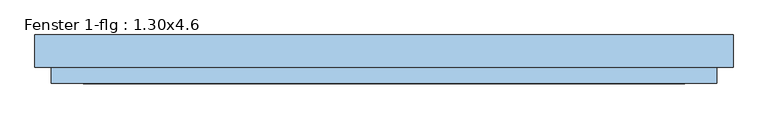
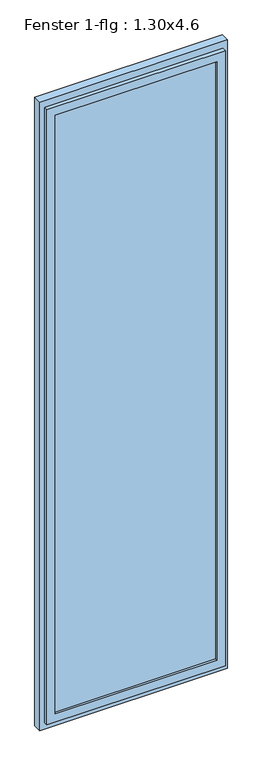
"""IFC4 building model written with IfcOpenShell, lengths in millimetres: window geometry, Fenster 1-flg : 1.30x4.6."""

from ifc_helpers import new_model, si_unit, frame, origin, place, context, project, spatial, polyline, outline, extrude, faceted_brep, source, transform, mapped, element, save


def fenster_1_flg_1_30x4_6_5ba6886f(model_context):
    return source(origin(), model_context, "Body", "SolidModel", [
        extrude(outline(polyline([(5600.0, 650.0), (5600.0, -650.0), (1000.0, -650.0), (1000.0, 650.0), (5600.0, 650.0)]), holes=[polyline([(5520.0, 590.0), (1080.0, 590.0), (1080.0, -590.0), (5520.0, -590.0), (5520.0, 590.0)])]), frame((0.0, -15.0, 0.0), z_axis=(0.0, 1.0, 0.0), x_axis=(0.0, 0.0, 1.0)), (0.0, 0.0, 1.0), 60.0),
        faceted_brep([(620.0, -15.0, 5550.0), (620.0, -45.0, 5550.0), (620.0, -45.0, 1050.0), (620.0, -15.0, 1050.0), (-620.0, -45.0, 5550.0), (-620.0, -45.0, 1050.0), (560.0, -45.0, 1110.0), (-560.0, -45.0, 1110.0), (-560.0, -45.0, 5490.0), (560.0, -45.0, 5490.0), (-620.0, -15.0, 1050.0), (-620.0, -15.0, 5550.0), (590.0, -15.0, 5520.0), (-590.0, -15.0, 5520.0), (-590.0, -15.0, 1080.0), (590.0, -15.0, 1080.0), (590.0, 15.0, 5520.0), (590.0, 15.0, 1080.0), (-590.0, 15.0, 1080.0), (-590.0, 15.0, 5520.0), (560.0, 15.0, 5490.0), (-560.0, 15.0, 5490.0), (-560.0, 15.0, 1110.0), (560.0, 15.0, 1110.0)], [[[0, 1, 2, 3]], [[1, 4, 5, 2], [6, 7, 8, 9]], [[3, 2, 5, 10]], [[3, 10, 11, 0], [12, 13, 14, 15]], [[16, 12, 15, 17]], [[17, 15, 14, 18]], [[17, 18, 19, 16], [20, 21, 22, 23]], [[9, 20, 23, 6]], [[6, 23, 22, 7]], [[10, 5, 4, 11]], [[18, 14, 13, 19]], [[7, 22, 21, 8]], [[11, 4, 1, 0]], [[19, 13, 12, 16]], [[8, 21, 20, 9]]]),
        extrude(outline(polyline([(560.0, -30.0), (-560.0, -30.0), (-560.0, 0.0), (560.0, 0.0), (560.0, -30.0)])), frame((0.0, 0.0, 1110.0), z_axis=(0.0, 0.0, 1.0), x_axis=(1.0, 0.0, 0.0)), (0.0, 0.0, 1.0), 4380.0),
    ])


if __name__ == "__main__":
    model = new_model("IFC4")
    model_context = context("Model", 3, world=origin())
    ifc_project = project(units=[si_unit("LENGTHUNIT", "METRE", prefix="MILLI")], contexts=[model_context])
    site = spatial("IfcSite", under=ifc_project)
    building = spatial("IfcBuilding", under=site)
    placement = place(None, origin())
    fenster_1_flg_1_30x4_6_shape = fenster_1_flg_1_30x4_6_5ba6886f(model_context)
    element("IfcWindow", 1, ObjectType="Fenster 1-flg : 1.30x4.6", at=placement, inside=building, context=model_context, shape_type="MappedRepresentation", body=[
        mapped(fenster_1_flg_1_30x4_6_shape, transform((0.0, 0.0, 0.0), x_axis=(1.0, 0.0, 0.0), y_axis=(0.0, 1.0, 0.0), z_axis=(0.0, 0.0, 1.0))),
    ])
    save(model, "model.ifc")

# Revit data of these elements
# Type "Fenster 1-flg : 1.30x4.6"
#   Type Mark = "79"
#   Operation = "SinglePanel"
#   Keynote = "16.05.01"
#   Visual Light Transmittance = 0.9
#   Solar Heat Gain Coefficient = 0.86
#   Rough Width = 1.300 m
#   Rough Height = 4.600 m
#   Heat Transfer Coefficient (U) = 5.5617 W/(m²·K)
#   Rahmentiefe = 0.060 m
#   Rahmenhöhe - unten = 0.080 m
#   Rahmenhöhe - oben = 0.080 m
#   Rahmenbreite = 0.060 m
#   Height = 4.600 m
#   Tiefe Flügel = 0.060 m
#   Flügelbreite = 0.060 m
#   Einbautiefe (von außen) [instance default] = 0.100 m
#   Width = 1.300 m
#   Klappflügel [instance default] = no
#   Kippflügel [instance default] = yes
#   Öffnungsrichtung in Draufsicht anzeigen [instance default] = no
#   Drehflügel 1 [instance default] = yes
#   Rahmen 1 [instance default] = none
#   Glas [instance default] = none
#   Flügel [instance default] = none
#   Fensterbank Innenseite [instance default] = none
#   Fensterbank Außenseite [instance default] = none
#   Construction Type Id = ""
#   Wall Closure = (empty or 0)
#   Analytic Construction = (empty or 0)
# Element 1 (IfcWindow, "Fenster 1-flg : 1.30x4.6")
#   Einbautiefe (von außen) = 0.230 m
#   Materials on its faces: "Kunststoff - Weiß", "Glas"
# Materials
#   "Kunststoff - Weiß": class "Kunststoff", colour RGB 249 249 249, transparency 0, Cost = 0
#   "Glas": class "Glas", colour RGB 0 0 255, transparency 0.75, Comments = "Render-Darstellung nicht aktualisiert ", Cost = 0
